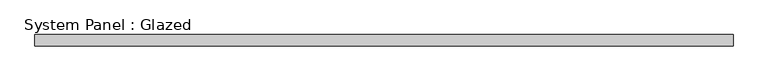
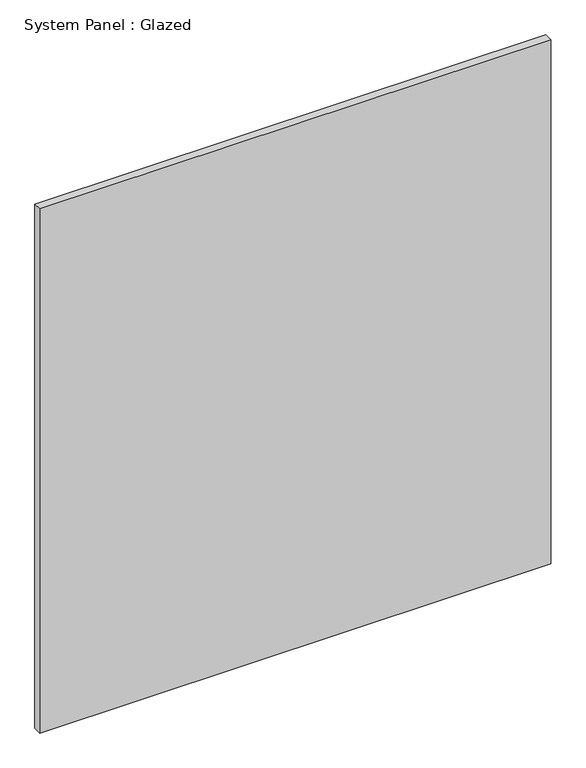
"""IFC4 building model written with IfcOpenShell, lengths in millimetres: plate geometry, System Panel : Glazed."""

from ifc_helpers import new_model, si_unit, origin, origin_with_axes, place, context, project, spatial, polyline, outline, extrude, source, transform, mapped, element, save


def system_panel_glazed_b93286e1(model_context):
    return source(origin(), model_context, "Body", "SweptSolid", [
        extrude(outline(polyline([(782.8178526, 24.5), (-782.8178526, 24.5), (-782.8178526, 49.5), (782.8178526, 49.5), (782.8178526, 24.5)])), origin_with_axes(), (0.0, 0.0, 1.0), 1698.3122923),
    ])


if __name__ == "__main__":
    model = new_model("IFC4")
    model_context = context("Model", 3, world=origin())
    ifc_project = project(units=[si_unit("LENGTHUNIT", "METRE", prefix="MILLI")], contexts=[model_context])
    site = spatial("IfcSite", under=ifc_project)
    building = spatial("IfcBuilding", under=site)
    placement = place(None, origin())
    system_panel_glazed_shape = system_panel_glazed_b93286e1(model_context)
    element("IfcPlate", 1, ObjectType="System Panel : Glazed", at=placement, inside=building, context=model_context, shape_type="MappedRepresentation", body=[
        mapped(system_panel_glazed_shape, transform((0.0, 0.0, 0.0), x_axis=(1.0, 0.0, 0.0), y_axis=(0.0, 1.0, 0.0), z_axis=(0.0, 0.0, 1.0))),
    ])
    save(model, "model.ifc")

# Revit data of these elements
# Element 1 (IfcPlate, "System Panel : Glazed")
#   Materials on its faces: "Glass"
# Materials
#   "Glass": class "Glass", colour RGB 218 227 224, transparency 0.85, Description = "Soda Lime Glass", Cost = 0
